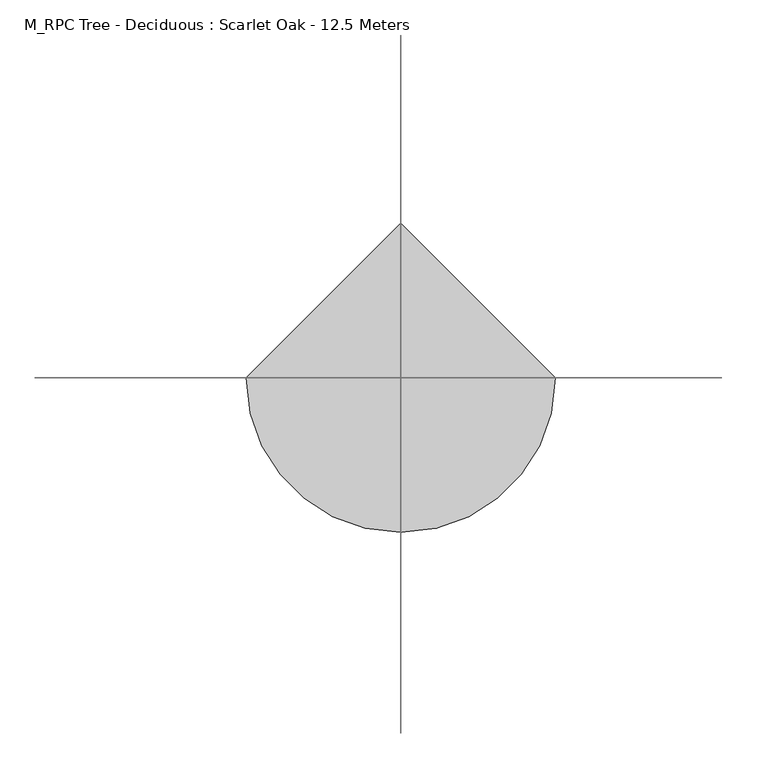
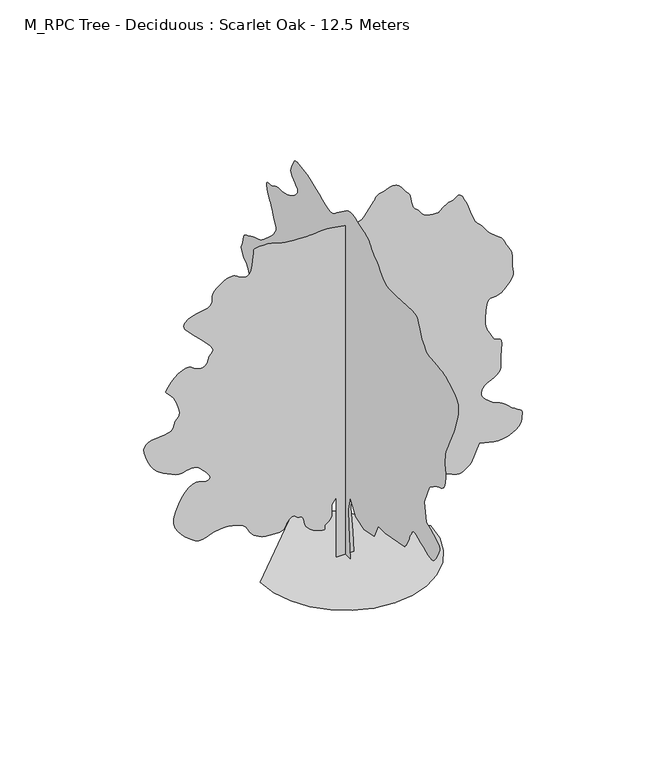
# IFC4 building model written with IfcOpenShell, lengths in millimetres: geographic element geometry, M_RPC Tree - Deciduous : Scarlet Oak - 12.5 Meters.
# Revit data of these elements (continued)
# Type "M_RPC Tree - Deciduous : Scarlet Oak - 12.5 Meters"
#   built-in parameter 1005198 = "{2, 15},{39, RPC-16-G0FB-J5PX-0LX6-U000-ST1L-LVER-AU},{1, 0},{1, 0},{2, 13},{1, 8},{5, Color},{1, 0},{1, 0},{3, 0.8},{3, 0.8},{3, 0.8},{1, 8},{7, BBoxMin},{1, 0},{1, 0},{1, 0},{1, 0},{1, 0},{1, 8},{7, BBoxMax},{1, 0},{1, 0},{1, 0},{1, 0},{1, 0},{2, 11},{9, RPCTypeId},{1, 0},{1, 0},{39, RPC-16-G0FB-J5PX-0LX6-U000-ST1L-LVER-AU},{1, 6},{14, RPCPlantHeight},{1, 0},{1, 0},{7, 41.0105},{2, 11},{7, keyword},{1, 0},{1, 0},{34, :RPCs:Trees [General]:Geometry:RPC},{2, 11},{8, category},{1, 0},{1, 0},{15, Trees [General]},{2, 11},{12, LocalizedUID},{1, 0},{1, 0},{11, Scarlet_Oak},{2, 14},{6, Height},{1, 0},{1, 0},{7, 41.0105},{1, 2},{16, Cast Reflections},{1, 0},{1, 0},{1, 0},{1, 2},{12, Cast Shadows},{1, 0},{1, 0},{1, 1},{1, 2},{9, Lock View},{1, 0},{1, 0},{1, 0},{1, 4},{5, ViewC},{1, 0},{1, 0},{1, 0},{21, assetlibrary_base.fbx},{1, 5},"
#   built-in parameter 1005195 = "RPC-16-G0FB-J5PX-0LX6-U000-ST1L-LVER-AU"
#   Type Comments = "Scarlet Oak"
#   Height = 12.50 m
